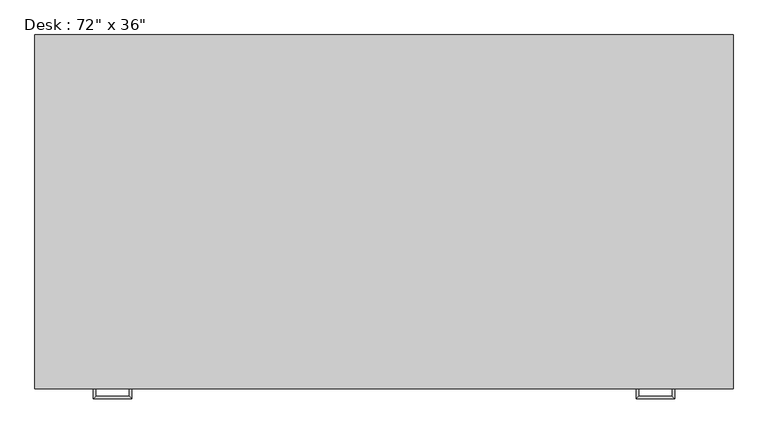
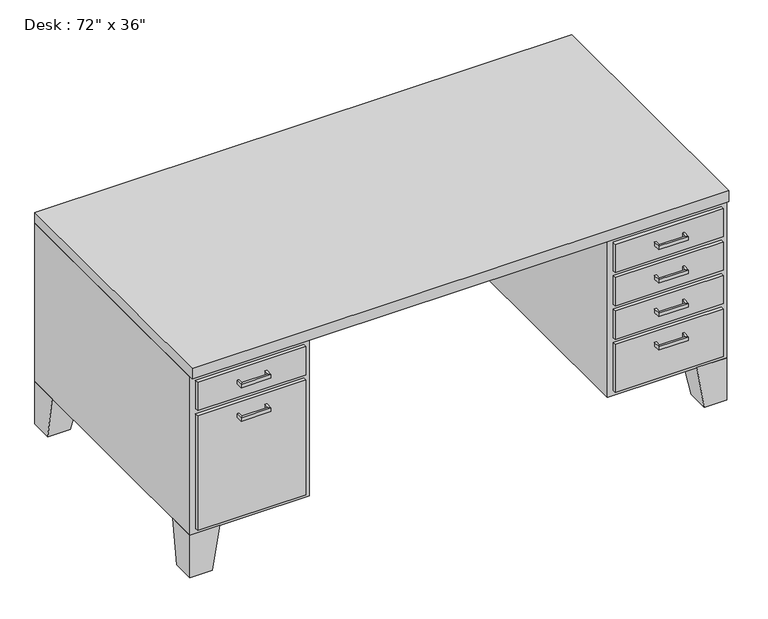
"""IFC4 building model written with IfcOpenShell, lengths in millimetres: furniture geometry."""

import ifcopenshell
import ifcopenshell.guid

model = None  # the IFC model being written
_history = None  # IfcOwnerHistory: only IFC2X3 demands one
_inside = {}  # id of a spatial element -> (the spatial element, [elements in it])
_under = {}  # id of a project, library or spatial element -> (it, [spatial elements below it])
_declared = {}  # id of a project -> (the project, [libraries it declares])
_typed = {}  # id of a type object -> (the type object, [elements of that type])
_made_of = {}  # id of a material, layer set ... -> (it, [elements and type objects made of it])


def new_model(schema):
    """Start an empty IFC model of exactly this schema.

    Asked for "IFC4X3", IfcOpenShell would pick the latest addendum, in which some entities
    have other attributes; the version numbers below select the first issue.
    IFC2X3 requires an IfcOwnerHistory on every rooted entity: one is made here for all.
    """
    global model, _history
    if schema == "IFC4X3":
        model = ifcopenshell.file(schema_version=(4, 3, 0, 0))
    else:
        model = ifcopenshell.file(schema=schema)
    _inside.clear()
    _under.clear()
    _declared.clear()
    _typed.clear()
    _made_of.clear()
    _history = None
    if model.schema == "IFC2X3":
        org = make("IfcOrganization", Name="unknown")
        user = make(
            "IfcPersonAndOrganization",
            ThePerson=make("IfcPerson", FamilyName="unknown"),
            TheOrganization=org,
        )
        app = make(
            "IfcApplication",
            ApplicationDeveloper=org,
            Version="unknown",
            ApplicationFullName="unknown",
            ApplicationIdentifier="unknown",
        )
        _history = make(
            "IfcOwnerHistory",
            OwningUser=user,
            OwningApplication=app,
            ChangeAction="ADDED",
            CreationDate=0,
        )
    return model


def make(cls, **values):
    """One entity of the class cls with the attributes given. An attribute that is None is left unset."""
    return model.create_entity(
        cls, **{name: value for name, value in values.items() if value is not None}
    )


def rooted(cls, **values):
    """An entity with a GlobalId (a new one), such as an element, a storey or a relation."""
    return make(cls, GlobalId=ifcopenshell.guid.new(), OwnerHistory=_history, **values)


def si_unit(unit_type, name, prefix=None):
    """IfcSIUnit, for example si_unit("LENGTHUNIT", "METRE", prefix="MILLI")."""
    return make("IfcSIUnit", UnitType=unit_type, Prefix=prefix, Name=name)


def assignment(units):
    """IfcUnitAssignment: the units of a project."""
    return None if units is None else make("IfcUnitAssignment", Units=units)


def point(xyz):
    """IfcCartesianPoint."""
    return None if xyz is None else make("IfcCartesianPoint", Coordinates=xyz)


def direction(xyz):
    """IfcDirection."""
    return None if xyz is None else make("IfcDirection", DirectionRatios=xyz)


def frame(location, z_axis=None, x_axis=None):
    """IfcAxis2Placement3D, a coordinate frame: its origin and axes. An axis left out is left unset."""
    return make(
        "IfcAxis2Placement3D",
        Location=point(location),
        Axis=direction(z_axis),
        RefDirection=direction(x_axis),
    )


def origin():
    """The frame at (0, 0, 0) with its axes left unset."""
    return frame((0.0, 0.0, 0.0))


def place(relative_to, where):
    """IfcLocalPlacement: puts the frame where relative to a parent placement (None: the world)."""
    return make(
        "IfcLocalPlacement", PlacementRelTo=relative_to, RelativePlacement=where
    )


def context(
    kind, dimensions, precision=None, world=None, true_north=None, identifier=None
):
    """IfcGeometricRepresentationContext, for example the 3D "Model" context."""
    return make(
        "IfcGeometricRepresentationContext",
        ContextIdentifier=identifier,
        ContextType=kind,
        CoordinateSpaceDimension=dimensions,
        Precision=precision,
        WorldCoordinateSystem=world,
        TrueNorth=true_north,
    )


def project(units=None, contexts=None):
    """IfcProject with its units and contexts."""
    return rooted(
        "IfcProject",
        Name="project",
        RepresentationContexts=contexts,
        UnitsInContext=assignment(units),
    )


def spatial(cls, under=None, at=None, **own):
    """A site, building, storey or space (cls), placed at a placement, below another one or the project."""
    s = rooted(cls, ObjectPlacement=at, **own)
    if under is not None:
        _under.setdefault(under.id(), (under, []))[1].append(s)
    return s


def polyline(points):
    """IfcPolyline through the points."""
    return make("IfcPolyline", Points=[point(p) for p in points])


def outline(outer, holes=None, kind="AREA"):
    """IfcArbitraryClosedProfileDef: a profile drawn as a closed curve; with holes, ...WithVoids."""
    if holes is None:
        return make("IfcArbitraryClosedProfileDef", ProfileType=kind, OuterCurve=outer)
    return make(
        "IfcArbitraryProfileDefWithVoids",
        ProfileType=kind,
        OuterCurve=outer,
        InnerCurves=holes,
    )


def extrude(swept, where, along, depth):
    """IfcExtrudedAreaSolid: the profile swept, set in the frame where, extruded along a direction by depth."""
    return make(
        "IfcExtrudedAreaSolid",
        SweptArea=swept,
        Position=where,
        ExtrudedDirection=direction(along),
        Depth=depth,
    )


def faces_of(points, faces, orient=None, outer=None):
    """IfcFace entities. A face is a list of loops; a loop is a list of indices into points, from 0.

    orient and outer hold one flag for each loop. By default every Orientation is true, the
    first loop of a face is its IfcFaceOuterBound and the others are IfcFaceBound.
    """
    made = []
    for i, loops in enumerate(faces):
        bounds = []
        for j, loop in enumerate(loops):
            is_outer = j == 0 if outer is None else outer[i][j]
            bounds.append(
                make(
                    "IfcFaceOuterBound" if is_outer else "IfcFaceBound",
                    Bound=make("IfcPolyLoop", Polygon=[points[k] for k in loop]),
                    Orientation=True if orient is None else orient[i][j],
                )
            )
        made.append(make("IfcFace", Bounds=bounds))
    return made


def faceted_brep(points, faces, orient=None, outer=None, voids=None):
    """IfcFacetedBrep: a solid bounded by flat faces; with voids (closed shells), ...WithVoids."""
    shared = [point(p) for p in points]
    hull = make("IfcClosedShell", CfsFaces=faces_of(shared, faces, orient, outer))
    if voids is None:
        return make("IfcFacetedBrep", Outer=hull)
    return make(
        "IfcFacetedBrepWithVoids",
        Outer=hull,
        Voids=[
            make(cls, CfsFaces=faces_of(shared, fs, o, b)) for cls, fs, o, b in voids
        ],
    )


def shape(context_of_items, identifier, shape_type, items):
    """IfcShapeRepresentation: the items that make up one representation, for example the "Body"."""
    return make(
        "IfcShapeRepresentation",
        ContextOfItems=context_of_items,
        RepresentationIdentifier=identifier,
        RepresentationType=shape_type,
        Items=items,
    )


def source(mapping_origin, context_of_items, identifier, shape_type, items):
    """IfcRepresentationMap: a shape defined once, which mapped items show again and again."""
    return make(
        "IfcRepresentationMap",
        MappingOrigin=mapping_origin,
        MappedRepresentation=shape(context_of_items, identifier, shape_type, items),
    )


def transform(
    local_origin,
    x_axis=None,
    y_axis=None,
    z_axis=None,
    scale=None,
    scale2=None,
    scale3=None,
    uniform=True,
):
    """IfcCartesianTransformationOperator3D, or its non-uniform kind. x_axis, y_axis, z_axis: its Axis1, 2, 3."""
    if uniform:
        return make(
            "IfcCartesianTransformationOperator3D",
            Axis1=direction(x_axis),
            Axis2=direction(y_axis),
            LocalOrigin=point(local_origin),
            Scale=scale,
            Axis3=direction(z_axis),
        )
    return make(
        "IfcCartesianTransformationOperator3DnonUniform",
        Axis1=direction(x_axis),
        Axis2=direction(y_axis),
        LocalOrigin=point(local_origin),
        Scale=scale,
        Axis3=direction(z_axis),
        Scale2=scale2,
        Scale3=scale3,
    )


def mapped(mapping_source, mapping_target):
    """IfcMappedItem: shows the shape of a source again, moved by a transform."""
    return make(
        "IfcMappedItem", MappingSource=mapping_source, MappingTarget=mapping_target
    )


def made_of(thing, what):
    """Note that an element or type object is made of a material, layer set ...; save() writes the relation."""
    if what is not None:
        _made_of.setdefault(what.id(), (what, []))[1].append(thing)
    return thing


def element(
    cls,
    number,
    at=None,
    inside=None,
    cuts=None,
    type_object=None,
    material=None,
    context=None,
    identifier="Body",
    shape_type=None,
    held_by="IfcProductDefinitionShape",
    body=None,
    shapes=None,
    **own,
):
    """One element of the class cls, such as IfcWall. Its Tag is "e" and its number.

    at: its placement. inside: the storey or other place that contains it. cuts: it is an
    opening in that element (IfcRelVoidsElement). A single representation is given by context,
    identifier, shape_type and body (its items); several are given by shapes. held_by: the class
    of the entity that holds the representations. save() writes the other relations.
    """
    e = rooted(cls, Tag="e%d" % number, ObjectPlacement=at, **own)
    if body is not None:
        shapes = [shape(context, identifier, shape_type, body)]
    if shapes is not None:
        e.Representation = make(held_by, Representations=shapes)
    if inside is not None:
        _inside.setdefault(inside.id(), (inside, []))[1].append(e)
    if cuts is not None:
        rooted(
            "IfcRelVoidsElement", RelatingBuildingElement=cuts, RelatedOpeningElement=e
        )
    if type_object is not None:
        _typed.setdefault(type_object.id(), (type_object, []))[1].append(e)
    return made_of(e, material)


def aggregate(whole, parts):
    """IfcRelAggregates: a whole, such as a stair, and the parts it consists of."""
    return rooted("IfcRelAggregates", RelatingObject=whole, RelatedObjects=parts)


def save(model, path):
    """Write the relations noted so far, then the file.

    IfcRelAggregates (storeys below a building ...), IfcRelContainedInSpatialStructure (elements
    in a storey), IfcRelDefinesByType, IfcRelAssociatesMaterial and IfcRelDeclares: one each for
    every whole, place, type object, material and project.
    """
    for whole, parts in _under.values():
        aggregate(whole, parts)
    for where, things in _inside.values():
        rooted(
            "IfcRelContainedInSpatialStructure",
            RelatedElements=things,
            RelatingStructure=where,
        )
    for kind, things in _typed.values():
        rooted("IfcRelDefinesByType", RelatedObjects=things, RelatingType=kind)
    for what, things in _made_of.values():
        rooted("IfcRelAssociatesMaterial", RelatedObjects=things, RelatingMaterial=what)
    for by, libraries in _declared.values():
        rooted("IfcRelDeclares", RelatingContext=by, RelatedDefinitions=libraries)
    model.write(path)


def furniture_33f25304(model_context):
    return source(origin(), model_context, "Body", "SolidModel", [
        extrude(outline(polyline([(-133.35, -76.2), (234.95, -76.2), (234.95, -88.9), (-133.35, -88.9), (-133.35, -76.2)])), frame((0.0, 0.0, 603.25), z_axis=(0.0, 0.0, 1.0), x_axis=(1.0, 0.0, 0.0)), (0.0, 0.0, 1.0), 101.6),
        extrude(outline(polyline([(-133.35, -76.2), (234.95, -76.2), (234.95, -88.9), (-133.35, -88.9), (-133.35, -76.2)])), frame((0.0, 0.0, 171.45), z_axis=(0.0, 0.0, 1.0), x_axis=(1.0, 0.0, 0.0)), (0.0, 0.0, 1.0), 412.75),
        extrude(outline(polyline([(1289.05, -76.2), (1657.35, -76.2), (1657.35, -88.9), (1289.05, -88.9), (1289.05, -76.2)])), frame((0.0, 0.0, 603.25), z_axis=(0.0, 0.0, 1.0), x_axis=(1.0, 0.0, 0.0)), (0.0, 0.0, 1.0), 101.6),
        extrude(outline(polyline([(1289.05, -76.2), (1657.35, -76.2), (1657.35, -88.9), (1289.05, -88.9), (1289.05, -76.2)])), frame((0.0, 0.0, 171.45), z_axis=(0.0, 0.0, 1.0), x_axis=(1.0, 0.0, 0.0)), (0.0, 0.0, 1.0), 171.45),
        extrude(outline(polyline([(1289.05, -76.2), (1657.35, -76.2), (1657.35, -88.9), (1289.05, -88.9), (1289.05, -76.2)])), frame((0.0, 0.0, 482.6), z_axis=(0.0, 0.0, 1.0), x_axis=(1.0, 0.0, 0.0)), (0.0, 0.0, 1.0), 101.6),
        extrude(outline(polyline([(1289.05, -76.2), (1657.35, -76.2), (1657.35, -88.9), (1289.05, -88.9), (1289.05, -76.2)])), frame((0.0, 0.0, 361.95), z_axis=(0.0, 0.0, 1.0), x_axis=(1.0, 0.0, 0.0)), (0.0, 0.0, 1.0), 101.6),
        faceted_brep([(-50.8, -76.2, 152.4), (-50.8, 25.4, 152.4), (-152.4, 25.4, 152.4), (-152.4, -76.2, 152.4), (-76.2, -76.2, 0.0), (-152.4, -76.2, 0.0), (-152.4, 0.0, 0.0), (-76.2, 0.0, 0.0)], [[[0, 1, 2, 3]], [[4, 5, 6, 7]], [[4, 7, 1, 0]], [[7, 6, 2, 1]], [[6, 5, 3, 2]], [[5, 4, 0, 3]]]),
        faceted_brep([(-50.8, 838.2, 152.4), (-152.4, 838.2, 152.4), (-152.4, 736.6, 152.4), (-50.8, 736.6, 152.4), (-76.2, 838.2, 0.0), (-76.2, 762.0, 0.0), (-152.4, 762.0, 0.0), (-152.4, 838.2, 0.0)], [[[0, 1, 2, 3]], [[4, 5, 6, 7]], [[4, 7, 1, 0]], [[7, 6, 2, 1]], [[6, 5, 3, 2]], [[5, 4, 0, 3]]]),
        faceted_brep([(1574.8, 838.2, 152.4), (1574.8, 736.6, 152.4), (1676.4, 736.6, 152.4), (1676.4, 838.2, 152.4), (1600.2, 838.2, 0.0), (1676.4, 838.2, 0.0), (1676.4, 762.0, 0.0), (1600.2, 762.0, 0.0)], [[[0, 1, 2, 3]], [[4, 5, 6, 7]], [[4, 7, 1, 0]], [[7, 6, 2, 1]], [[6, 5, 3, 2]], [[5, 4, 0, 3]]]),
        faceted_brep([(1574.8, -76.2, 152.4), (1676.4, -76.2, 152.4), (1676.4, 25.4, 152.4), (1574.8, 25.4, 152.4), (1600.2, -76.2, 0.0), (1600.2, 0.0, 0.0), (1676.4, 0.0, 0.0), (1676.4, -76.2, 0.0)], [[[0, 1, 2, 3]], [[4, 5, 6, 7]], [[4, 7, 1, 0]], [[7, 6, 2, 1]], [[6, 5, 3, 2]], [[5, 4, 0, 3]]]),
        extrude(outline(polyline([(-152.4, -88.9), (-152.4, 838.2), (1676.4, 838.2), (1676.4, -88.9), (-152.4, -88.9)])), frame((0.0, 0.0, 723.9), z_axis=(0.0, 0.0, 1.0), x_axis=(1.0, 0.0, 0.0)), (0.0, 0.0, 1.0), 38.1),
        extrude(outline(polyline([(1270.0, -76.2), (1270.0, 711.2), (254.0, 711.2), (254.0, -76.2), (-152.4, -76.2), (-152.4, 838.2), (1676.4, 838.2), (1676.4, -76.2), (1270.0, -76.2)])), frame((0.0, 0.0, 152.4), z_axis=(0.0, 0.0, 1.0), x_axis=(1.0, 0.0, 0.0)), (0.0, 0.0, 1.0), 571.5),
        faceted_brep([(6.35, -88.9, 546.1), (6.35, -88.9, 533.4), (0.0, -88.9, 533.4), (0.0, -88.9, 546.1), (6.35, -107.95, 546.1), (6.35, -107.95, 533.4), (0.0, -114.3, 533.4), (0.0, -114.3, 546.1), (95.25, -107.95, 546.1), (95.25, -107.95, 533.4), (101.6, -114.3, 533.4), (101.6, -114.3, 546.1), (95.25, -88.9, 546.1), (101.6, -88.9, 546.1), (101.6, -88.9, 533.4), (95.25, -88.9, 533.4)], [[[0, 1, 2, 3]], [[1, 0, 4, 5]], [[2, 1, 5, 6]], [[3, 2, 6, 7]], [[0, 3, 7, 4]], [[5, 4, 8, 9]], [[6, 5, 9, 10]], [[7, 6, 10, 11]], [[4, 7, 11, 8]], [[12, 13, 14, 15]], [[9, 8, 12, 15]], [[10, 9, 15, 14]], [[11, 10, 14, 13]], [[8, 11, 13, 12]]]),
        faceted_brep([(6.35, -88.9, 666.75), (6.35, -88.9, 654.05), (0.0, -88.9, 654.05), (0.0, -88.9, 666.75), (6.35, -107.95, 666.75), (6.35, -107.95, 654.05), (0.0, -114.3, 654.05), (0.0, -114.3, 666.75), (95.25, -107.95, 666.75), (95.25, -107.95, 654.05), (101.6, -114.3, 654.05), (101.6, -114.3, 666.75), (95.25, -88.9, 666.75), (101.6, -88.9, 666.75), (101.6, -88.9, 654.05), (95.25, -88.9, 654.05)], [[[0, 1, 2, 3]], [[1, 0, 4, 5]], [[2, 1, 5, 6]], [[3, 2, 6, 7]], [[0, 3, 7, 4]], [[5, 4, 8, 9]], [[6, 5, 9, 10]], [[7, 6, 10, 11]], [[4, 7, 11, 8]], [[12, 13, 14, 15]], [[9, 8, 12, 15]], [[10, 9, 15, 14]], [[11, 10, 14, 13]], [[8, 11, 13, 12]]]),
        faceted_brep([(1517.65, -88.9, 304.8), (1524.0, -88.9, 304.8), (1524.0, -88.9, 292.1), (1517.65, -88.9, 292.1), (1517.65, -107.95, 304.8), (1524.0, -114.3, 304.8), (1524.0, -114.3, 292.1), (1517.65, -107.95, 292.1), (1428.75, -107.95, 304.8), (1422.4, -114.3, 304.8), (1422.4, -114.3, 292.1), (1428.75, -107.95, 292.1), (1428.75, -88.9, 304.8), (1428.75, -88.9, 292.1), (1422.4, -88.9, 292.1), (1422.4, -88.9, 304.8)], [[[0, 1, 2, 3]], [[1, 0, 4, 5]], [[2, 1, 5, 6]], [[3, 2, 6, 7]], [[0, 3, 7, 4]], [[5, 4, 8, 9]], [[6, 5, 9, 10]], [[7, 6, 10, 11]], [[4, 7, 11, 8]], [[12, 13, 14, 15]], [[9, 8, 12, 15]], [[10, 9, 15, 14]], [[11, 10, 14, 13]], [[8, 11, 13, 12]]]),
        faceted_brep([(1517.65, -88.9, 425.45), (1524.0, -88.9, 425.45), (1524.0, -88.9, 412.75), (1517.65, -88.9, 412.75), (1517.65, -107.95, 425.45), (1524.0, -114.3, 425.45), (1524.0, -114.3, 412.75), (1517.65, -107.95, 412.75), (1428.75, -107.95, 425.45), (1422.4, -114.3, 425.45), (1422.4, -114.3, 412.75), (1428.75, -107.95, 412.75), (1428.75, -88.9, 425.45), (1428.75, -88.9, 412.75), (1422.4, -88.9, 412.75), (1422.4, -88.9, 425.45)], [[[0, 1, 2, 3]], [[1, 0, 4, 5]], [[2, 1, 5, 6]], [[3, 2, 6, 7]], [[0, 3, 7, 4]], [[5, 4, 8, 9]], [[6, 5, 9, 10]], [[7, 6, 10, 11]], [[4, 7, 11, 8]], [[12, 13, 14, 15]], [[9, 8, 12, 15]], [[10, 9, 15, 14]], [[11, 10, 14, 13]], [[8, 11, 13, 12]]]),
        faceted_brep([(1517.65, -88.9, 546.1), (1524.0, -88.9, 546.1), (1524.0, -88.9, 533.4), (1517.65, -88.9, 533.4), (1517.65, -107.95, 546.1), (1524.0, -114.3, 546.1), (1524.0, -114.3, 533.4), (1517.65, -107.95, 533.4), (1428.75, -107.95, 546.1), (1422.4, -114.3, 546.1), (1422.4, -114.3, 533.4), (1428.75, -107.95, 533.4), (1428.75, -88.9, 546.1), (1428.75, -88.9, 533.4), (1422.4, -88.9, 533.4), (1422.4, -88.9, 546.1)], [[[0, 1, 2, 3]], [[1, 0, 4, 5]], [[2, 1, 5, 6]], [[3, 2, 6, 7]], [[0, 3, 7, 4]], [[5, 4, 8, 9]], [[6, 5, 9, 10]], [[7, 6, 10, 11]], [[4, 7, 11, 8]], [[12, 13, 14, 15]], [[9, 8, 12, 15]], [[10, 9, 15, 14]], [[11, 10, 14, 13]], [[8, 11, 13, 12]]]),
        faceted_brep([(1517.65, -88.9, 666.75), (1524.0, -88.9, 666.75), (1524.0, -88.9, 654.05), (1517.65, -88.9, 654.05), (1517.65, -107.95, 666.75), (1524.0, -114.3, 666.75), (1524.0, -114.3, 654.05), (1517.65, -107.95, 654.05), (1428.75, -107.95, 666.75), (1422.4, -114.3, 666.75), (1422.4, -114.3, 654.05), (1428.75, -107.95, 654.05), (1428.75, -88.9, 666.75), (1428.75, -88.9, 654.05), (1422.4, -88.9, 654.05), (1422.4, -88.9, 666.75)], [[[0, 1, 2, 3]], [[1, 0, 4, 5]], [[2, 1, 5, 6]], [[3, 2, 6, 7]], [[0, 3, 7, 4]], [[5, 4, 8, 9]], [[6, 5, 9, 10]], [[7, 6, 10, 11]], [[4, 7, 11, 8]], [[12, 13, 14, 15]], [[9, 8, 12, 15]], [[10, 9, 15, 14]], [[11, 10, 14, 13]], [[8, 11, 13, 12]]]),
    ])


if __name__ == "__main__":
    model = new_model("IFC4")
    model_context = context("Model", 3, world=origin())
    ifc_project = project(units=[si_unit("LENGTHUNIT", "METRE", prefix="MILLI")], contexts=[model_context])
    site = spatial("IfcSite", under=ifc_project)
    building = spatial("IfcBuilding", under=site)
    placement = place(None, origin())
    furniture_shape = furniture_33f25304(model_context)
    element("IfcFurniture", 1, ObjectType="Desk : 72\" x 36\"", at=placement, inside=building, context=model_context, shape_type="MappedRepresentation", body=[
        mapped(furniture_shape, transform((0.0, 0.0, 0.0), x_axis=(1.0, 0.0, 0.0), y_axis=(0.0, 1.0, 0.0), z_axis=(0.0, 0.0, 1.0))),
    ])
    save(model, "model.ifc")

# Revit data of these elements
# Type "Desk : 72\" x 36\""
#   Assembly Code = "E2020200"
#   Depth = 3' - 0"
#   Height = 2' - 6"
#   Leg Height = 0' - 6"
#   Width = 6' - 0"
#   Body Material = Laminate, Ivory, Matte
#   Handle/Leg Material = Steel, Chrome Plated
#   Top Material = Cherry
#   Default Elevation = 0
# Element 1 (IfcFurniture, "Desk : 72\" x 36\"")
#   Materials on its faces: "Steel, Chrome Plated", "Laminate, Ivory, Matte", "Cherry"
# Materials
#   "Laminate, Ivory, Matte": class "Plastic", colour RGB 247 247 239, transparency 0, Description = "Plastic Laminate - Ivory, Matte", Cost = 0
#   "Steel, Chrome Plated": class "Metal", colour RGB 17 17 17, transparency 0, Description = "Chromiuim plated steel", Cost = 0
#   "Cherry": class "Wood", colour RGB 226 177 128, transparency 0, Description = "Prunus Serotina", Cost = 0
